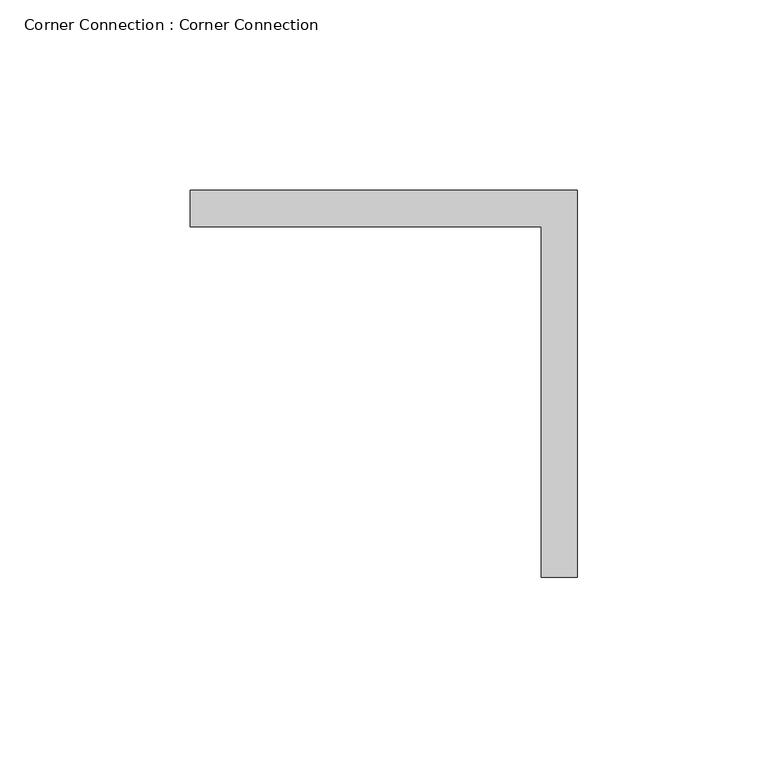
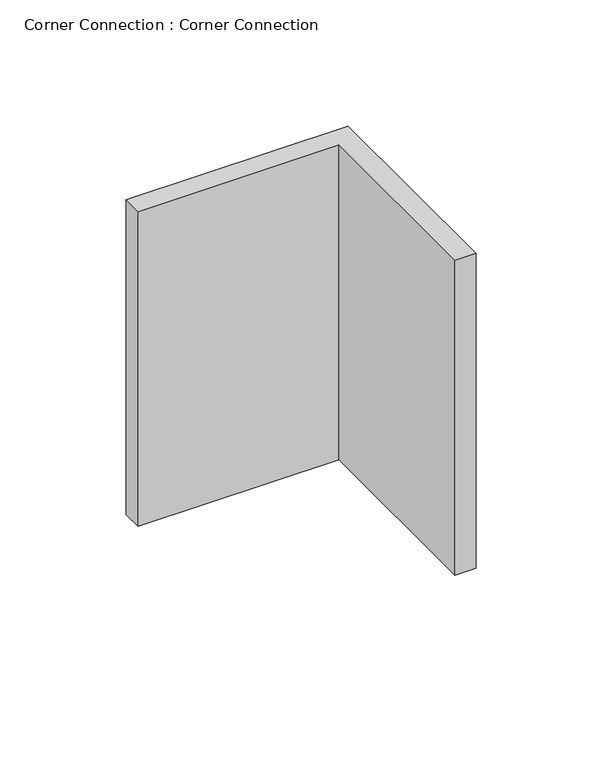
"""IFC4 building model written with IfcOpenShell, lengths in millimetres: fastener geometry, Corner Connection : Corner Connection."""

from ifc_helpers import new_model, si_unit, origin, origin_with_axes, place, context, project, spatial, polyline, outline, extrude, source, transform, mapped, element, save


def corner_connection_corner_connection_f308c9d5(model_context):
    return source(origin(), model_context, "Body", "SweptSolid", [
        extrude(outline(polyline([(-101.6, 0.0), (0.0, 0.0), (0.0, -101.6), (-9.525, -101.6), (-9.525, -9.525), (-101.6, -9.525), (-101.6, 0.0)])), origin_with_axes(), (0.0, 0.0, 1.0), 152.4),
    ])


if __name__ == "__main__":
    model = new_model("IFC4")
    model_context = context("Model", 3, world=origin())
    ifc_project = project(units=[si_unit("LENGTHUNIT", "METRE", prefix="MILLI")], contexts=[model_context])
    site = spatial("IfcSite", under=ifc_project)
    building = spatial("IfcBuilding", under=site)
    placement = place(None, origin())
    corner_connection_corner_connection_shape = corner_connection_corner_connection_f308c9d5(model_context)
    element("IfcFastener", 1, ObjectType="Corner Connection : Corner Connection", at=placement, inside=building, context=model_context, shape_type="MappedRepresentation", body=[
        mapped(corner_connection_corner_connection_shape, transform((0.0, 0.0, 0.0), x_axis=(1.0, 0.0, 0.0), y_axis=(0.0, 1.0, 0.0), z_axis=(0.0, 0.0, 1.0))),
    ])
    save(model, "model.ifc")

# Revit data of these elements
# Type "Corner Connection : Corner Connection"
#   MATERIAL = Galvanized Steel
# Element 1 (IfcFastener, "Corner Connection : Corner Connection")
#   Materials on its faces: "Galvanized Steel"
# Materials
#   "Galvanized Steel": class "Generic", colour RGB 232 232 232, transparency 0, Description = "Acoustic Ceiling Tile 24 x 24", Cost = 0
